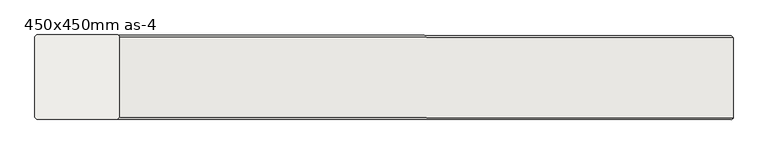
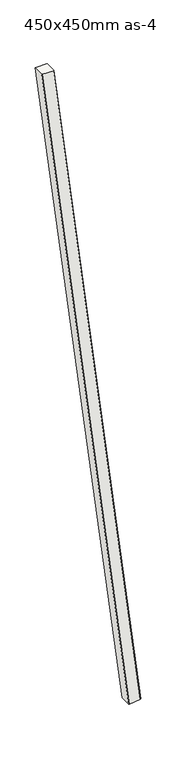
"""IFC4 building model written with IfcOpenShell, lengths in millimetres: slab geometry, CO_01_001_Geheide_prefab_betonpaal : 450x450mm as-4."""

from ifc_helpers import new_model, si_unit, origin, place, context, project, spatial, faceted_brep, source, transform, mapped, element, save


def slab_450x450mm_as_4_7009cd29(model_context):
    return source(origin(), model_context, "Body", "Brep", [
        faceted_brep([(3494.5897435, -225.0, -22473.3325321), (3067.9102565, -225.0, -22526.6674679), (3057.9874777, -215.0, -22527.9078153), (3057.9874777, 215.0, -22527.9078153), (3067.9102565, 225.0, -22526.6674679), (3494.5897435, 225.0, -22473.3325321), (3504.5125223, 215.0, -22472.0921847), (3504.5125223, -215.0, -22472.0921847), (226.7509992, -215.0, 3750.0), (216.673177, -225.0, 3750.0), (226.7509992, 215.0, 3750.0), (216.673177, 225.0, 3750.0), (-216.673177, 225.0, 3750.0), (-226.7509992, 215.0, 3750.0), (-226.7509992, -215.0, 3750.0), (-216.673177, -225.0, 3750.0)], [[[0, 1, 2, 3, 4, 5, 6, 7]], [[0, 7, 8, 9]], [[7, 6, 10, 8]], [[6, 5, 11, 10]], [[5, 4, 12, 11]], [[4, 3, 13, 12]], [[3, 2, 14, 13]], [[2, 1, 15, 14]], [[1, 0, 9, 15]], [[9, 8, 10, 11, 12, 13, 14, 15]]]),
    ])


if __name__ == "__main__":
    model = new_model("IFC4")
    model_context = context("Model", 3, world=origin())
    ifc_project = project(units=[si_unit("LENGTHUNIT", "METRE", prefix="MILLI")], contexts=[model_context])
    site = spatial("IfcSite", under=ifc_project)
    building = spatial("IfcBuilding", under=site)
    placement = place(None, origin())
    slab_450x450mm_as_4_shape = slab_450x450mm_as_4_7009cd29(model_context)
    element("IfcSlab", 1, ObjectType="CO_01_001_Geheide_prefab_betonpaal : 450x450mm as-4", at=placement, inside=building, context=model_context, shape_type="MappedRepresentation", body=[
        mapped(slab_450x450mm_as_4_shape, transform((0.0, 0.0, 0.0), x_axis=(1.0, 0.0, 0.0), y_axis=(0.0, 1.0, 0.0), z_axis=(0.0, 0.0, 1.0))),
    ])
    save(model, "model.ifc")

# Revit data of these elements
# Type "CO_01_001_Geheide_prefab_betonpaal : 450x450mm as-4"
#   Omschrijving = "Geheide prefab betonpaal; 450x450mm"
#   Description = "Driven precast concrete pile; 450x450mm"
#   CHECK_paallengte [instance default] = "geen problemen"
#   CHECK_raker [instance default] = "geen problemen"
#   Assembly Code = "CO_01_001"
#   Schoorstand_.._1 [instance default] = 5
#   Max_lengte = 37000 mm
#   CALC_WidthNeg [instance default] = -450 mm
#   Width = 450 mm
#   CALC_Vert Pile Length [instance default] = 2250 mm
#   Vellingkant = 10 mm
#   CALC_Top Level [instance default] = 150 mm
#   CALC_asInput_ToeLevel [instance default] = 2250 mm
#   Schoorstand_graden [instance default] = 78.6901°
#   Schoorstand_1_ [instance default] = 0.2
#   Onderkant [instance default] = -1500 mm
#   Lengte [instance default] = 2549.51 mm
#   Bovenkant_tov_NAP [instance default] = 1000 mm
#   Onderkant_tov_NAP [instance default] = -1500 mm
#   CALC_Slopedist cut off [instance default] = 50.99 mm
#   CALC_Slopedist bottom [instance default] = 450 mm
#   CALC_Slopedist Toe Level [instance default] = 450 mm
#   CALC_Slopedist Pile length [instance default] = 450 mm
#   CALC_Refplane Top [instance default] = 900 mm
#   CALC_Rakersymbol rotation [instance default] = 90.00°
#   Schoorsymbool_rotatie [instance default] = 0.00°
#   CALC_Rakersymbol Offset [instance default] = 225 mm
#   CALC_asInput_PileLength [instance default] = -254.951 mm
#   Lengte_paal [instance default] = 0 mm
#   CALC_FlatcutExtention_height [instance default] = 112.5 mm
#   CALC_FlatcutExtention_dist [instance default] = 22.5 mm
#   CALC_CutOff [instance default] = 254.951 mm
#   Bovenkant [instance default] = 1000 mm
#   Afhak_hoogte_tov_NAP [instance default] = 750 mm
#   Rakertext Rotate 90deg [instance default] = no
#   Rakertext Rotate 270deg [instance default] = no
#   Rakertext Rotate 180deg [instance default] = no
#   Rakertext Rotate 0deg [instance default] = yes
#   RakerSymbol_vis [instance default] = yes
#   Paal_per_lengte [instance default] = no
#   Cut off_vis [instance default] = yes
#   Pile Symbol = element 2909617
#   Structural Material = none
#   Length = 0
# Element 1 (IfcSlab, "CO_01_001_Geheide_prefab_betonpaal : 450x450mm as-4")
#   Schoorstand_.._1 = 8
#   CALC_Vert Pile Length = 26250 mm
#   CALC_asInput_ToeLevel = 26250 mm
#   Schoorstand_graden = 82.875°
#   Schoorstand_1_ = 0.125
#   Onderkant = -22500 mm
#   Lengte = 26454.283 mm
#   Bovenkant_tov_NAP = 3750 mm
#   Onderkant_tov_NAP = -22500 mm
#   CALC_Slopedist cut off = 0 mm
#   CALC_Slopedist bottom = 3281.25 mm
#   CALC_Slopedist Toe Level = 3281.25 mm
#   CALC_Slopedist Pile length = 3281.25 mm
#   CALC_Refplane Top = 3900 mm
#   CALC_asInput_PileLength = 0 mm
#   CALC_FlatcutExtention_dist = 14.063 mm
#   CALC_CutOff = 0 mm
#   Bovenkant = 3750 mm
#   Afhak_hoogte_tov_NAP = 3750 mm
#   Cut off_vis = no
#   Materials on its faces: "Beton_Prefab"
# Materials
#   "Beton_Prefab": class "Beton", colour RGB 192 192 192, transparency 0, Description = "NL_Infra", Cost = 0
